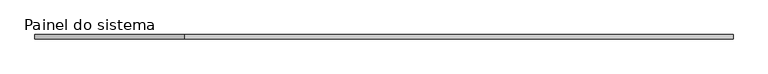
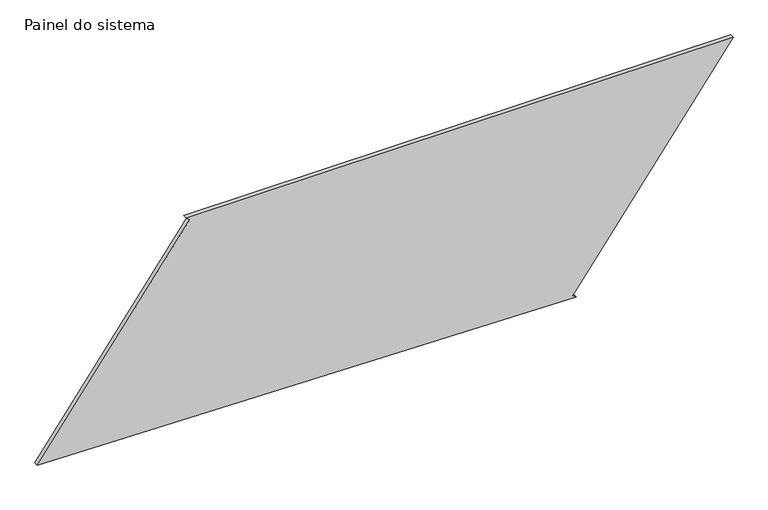
"""IFC4 building model written with IfcOpenShell, lengths in millimetres: plate geometry, Painel do sistema : Envidraçado."""

from ifc_helpers import new_model, si_unit, frame, origin, place, context, project, spatial, polyline, outline, extrude, source, transform, mapped, element, save


def painel_do_sistema_59cc7aff(model_context):
    return source(origin(), model_context, "Body", "SweptSolid", [
        extrude(outline(polyline([(0.0, 1107.3370957), (14.8374505, 1087.2162095), (1272.1486312, 2014.3767811), (1272.1486312, -1151.0267052), (1257.3111807, -1130.905819), (59.2469484, -2014.3767811), (0.0, 1107.3370957)])), frame((0.0, 24.5, 0.0), z_axis=(0.0, 1.0, 0.0), x_axis=(0.0, 0.0, 1.0)), (0.0, 0.0, 1.0), 25.0),
    ])


if __name__ == "__main__":
    model = new_model("IFC4")
    model_context = context("Model", 3, world=origin())
    ifc_project = project(units=[si_unit("LENGTHUNIT", "METRE", prefix="MILLI")], contexts=[model_context])
    site = spatial("IfcSite", under=ifc_project)
    building = spatial("IfcBuilding", under=site)
    placement = place(None, origin())
    painel_do_sistema_shape = painel_do_sistema_59cc7aff(model_context)
    element("IfcPlate", 1, ObjectType="Painel do sistema : Envidraçado", at=placement, inside=building, context=model_context, shape_type="MappedRepresentation", body=[
        mapped(painel_do_sistema_shape, transform((0.0, 0.0, 0.0), x_axis=(1.0, 0.0, 0.0), y_axis=(0.0, 1.0, 0.0), z_axis=(0.0, 0.0, 1.0))),
    ])
    save(model, "model.ifc")

# Revit data of these elements
# Type "Painel do sistema : Envidraçado"
#   Construction Type Id = "GSP4R"
#   Analytic Construction = "Vidraça única Pilkington 1/8 pol"
#   Visual Light Transmittance = 0.9
#   Solar Heat Gain Coefficient = 0.86
#   Heat Transfer Coefficient (U) = 6.7069 W/(m²·K)
# Element 1 (IfcPlate, "Painel do sistema : Envidraçado")
#   Materials on its faces: "Vidro"
# Materials
#   "Vidro": class "Vidro", colour RGB 0 128 192, transparency 0.9, Description = "Vidro de sílica", Cost = 0
